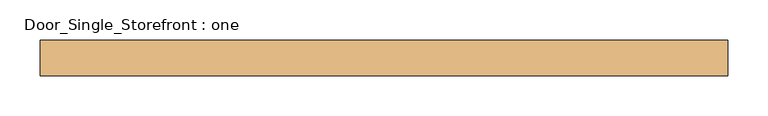
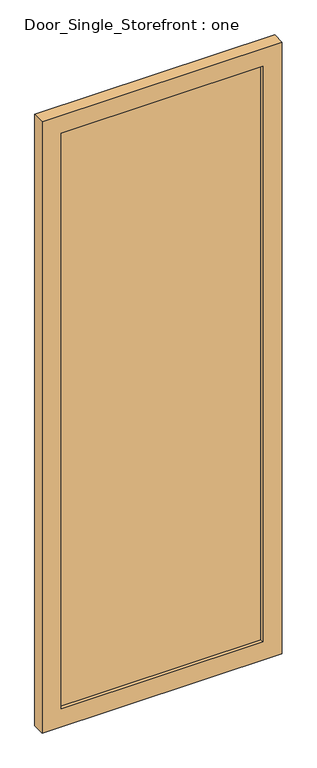
"""IFC4 building model written with IfcOpenShell, lengths in millimetres: door geometry, Door_Single_Storefront : one."""

import ifcopenshell
import ifcopenshell.guid

model = None  # the IFC model being written
_history = None  # IfcOwnerHistory: only IFC2X3 demands one
_inside = {}  # id of a spatial element -> (the spatial element, [elements in it])
_under = {}  # id of a project, library or spatial element -> (it, [spatial elements below it])
_declared = {}  # id of a project -> (the project, [libraries it declares])
_typed = {}  # id of a type object -> (the type object, [elements of that type])
_made_of = {}  # id of a material, layer set ... -> (it, [elements and type objects made of it])


def new_model(schema):
    """Start an empty IFC model of exactly this schema.

    Asked for "IFC4X3", IfcOpenShell would pick the latest addendum, in which some entities
    have other attributes; the version numbers below select the first issue.
    IFC2X3 requires an IfcOwnerHistory on every rooted entity: one is made here for all.
    """
    global model, _history
    if schema == "IFC4X3":
        model = ifcopenshell.file(schema_version=(4, 3, 0, 0))
    else:
        model = ifcopenshell.file(schema=schema)
    _inside.clear()
    _under.clear()
    _declared.clear()
    _typed.clear()
    _made_of.clear()
    _history = None
    if model.schema == "IFC2X3":
        org = make("IfcOrganization", Name="unknown")
        user = make(
            "IfcPersonAndOrganization",
            ThePerson=make("IfcPerson", FamilyName="unknown"),
            TheOrganization=org,
        )
        app = make(
            "IfcApplication",
            ApplicationDeveloper=org,
            Version="unknown",
            ApplicationFullName="unknown",
            ApplicationIdentifier="unknown",
        )
        _history = make(
            "IfcOwnerHistory",
            OwningUser=user,
            OwningApplication=app,
            ChangeAction="ADDED",
            CreationDate=0,
        )
    return model


def make(cls, **values):
    """One entity of the class cls with the attributes given. An attribute that is None is left unset."""
    return model.create_entity(
        cls, **{name: value for name, value in values.items() if value is not None}
    )


def rooted(cls, **values):
    """An entity with a GlobalId (a new one), such as an element, a storey or a relation."""
    return make(cls, GlobalId=ifcopenshell.guid.new(), OwnerHistory=_history, **values)


def si_unit(unit_type, name, prefix=None):
    """IfcSIUnit, for example si_unit("LENGTHUNIT", "METRE", prefix="MILLI")."""
    return make("IfcSIUnit", UnitType=unit_type, Prefix=prefix, Name=name)


def assignment(units):
    """IfcUnitAssignment: the units of a project."""
    return None if units is None else make("IfcUnitAssignment", Units=units)


def point(xyz):
    """IfcCartesianPoint."""
    return None if xyz is None else make("IfcCartesianPoint", Coordinates=xyz)


def direction(xyz):
    """IfcDirection."""
    return None if xyz is None else make("IfcDirection", DirectionRatios=xyz)


def frame(location, z_axis=None, x_axis=None):
    """IfcAxis2Placement3D, a coordinate frame: its origin and axes. An axis left out is left unset."""
    return make(
        "IfcAxis2Placement3D",
        Location=point(location),
        Axis=direction(z_axis),
        RefDirection=direction(x_axis),
    )


def origin():
    """The frame at (0, 0, 0) with its axes left unset."""
    return frame((0.0, 0.0, 0.0))


def place(relative_to, where):
    """IfcLocalPlacement: puts the frame where relative to a parent placement (None: the world)."""
    return make(
        "IfcLocalPlacement", PlacementRelTo=relative_to, RelativePlacement=where
    )


def context(
    kind, dimensions, precision=None, world=None, true_north=None, identifier=None
):
    """IfcGeometricRepresentationContext, for example the 3D "Model" context."""
    return make(
        "IfcGeometricRepresentationContext",
        ContextIdentifier=identifier,
        ContextType=kind,
        CoordinateSpaceDimension=dimensions,
        Precision=precision,
        WorldCoordinateSystem=world,
        TrueNorth=true_north,
    )


def project(units=None, contexts=None):
    """IfcProject with its units and contexts."""
    return rooted(
        "IfcProject",
        Name="project",
        RepresentationContexts=contexts,
        UnitsInContext=assignment(units),
    )


def spatial(cls, under=None, at=None, **own):
    """A site, building, storey or space (cls), placed at a placement, below another one or the project."""
    s = rooted(cls, ObjectPlacement=at, **own)
    if under is not None:
        _under.setdefault(under.id(), (under, []))[1].append(s)
    return s


def polyline(points):
    """IfcPolyline through the points."""
    return make("IfcPolyline", Points=[point(p) for p in points])


def outline(outer, holes=None, kind="AREA"):
    """IfcArbitraryClosedProfileDef: a profile drawn as a closed curve; with holes, ...WithVoids."""
    if holes is None:
        return make("IfcArbitraryClosedProfileDef", ProfileType=kind, OuterCurve=outer)
    return make(
        "IfcArbitraryProfileDefWithVoids",
        ProfileType=kind,
        OuterCurve=outer,
        InnerCurves=holes,
    )


def extrude(swept, where, along, depth):
    """IfcExtrudedAreaSolid: the profile swept, set in the frame where, extruded along a direction by depth."""
    return make(
        "IfcExtrudedAreaSolid",
        SweptArea=swept,
        Position=where,
        ExtrudedDirection=direction(along),
        Depth=depth,
    )


def shape(context_of_items, identifier, shape_type, items):
    """IfcShapeRepresentation: the items that make up one representation, for example the "Body"."""
    return make(
        "IfcShapeRepresentation",
        ContextOfItems=context_of_items,
        RepresentationIdentifier=identifier,
        RepresentationType=shape_type,
        Items=items,
    )


def source(mapping_origin, context_of_items, identifier, shape_type, items):
    """IfcRepresentationMap: a shape defined once, which mapped items show again and again."""
    return make(
        "IfcRepresentationMap",
        MappingOrigin=mapping_origin,
        MappedRepresentation=shape(context_of_items, identifier, shape_type, items),
    )


def transform(
    local_origin,
    x_axis=None,
    y_axis=None,
    z_axis=None,
    scale=None,
    scale2=None,
    scale3=None,
    uniform=True,
):
    """IfcCartesianTransformationOperator3D, or its non-uniform kind. x_axis, y_axis, z_axis: its Axis1, 2, 3."""
    if uniform:
        return make(
            "IfcCartesianTransformationOperator3D",
            Axis1=direction(x_axis),
            Axis2=direction(y_axis),
            LocalOrigin=point(local_origin),
            Scale=scale,
            Axis3=direction(z_axis),
        )
    return make(
        "IfcCartesianTransformationOperator3DnonUniform",
        Axis1=direction(x_axis),
        Axis2=direction(y_axis),
        LocalOrigin=point(local_origin),
        Scale=scale,
        Axis3=direction(z_axis),
        Scale2=scale2,
        Scale3=scale3,
    )


def mapped(mapping_source, mapping_target):
    """IfcMappedItem: shows the shape of a source again, moved by a transform."""
    return make(
        "IfcMappedItem", MappingSource=mapping_source, MappingTarget=mapping_target
    )


def made_of(thing, what):
    """Note that an element or type object is made of a material, layer set ...; save() writes the relation."""
    if what is not None:
        _made_of.setdefault(what.id(), (what, []))[1].append(thing)
    return thing


def element(
    cls,
    number,
    at=None,
    inside=None,
    cuts=None,
    type_object=None,
    material=None,
    context=None,
    identifier="Body",
    shape_type=None,
    held_by="IfcProductDefinitionShape",
    body=None,
    shapes=None,
    **own,
):
    """One element of the class cls, such as IfcWall. Its Tag is "e" and its number.

    at: its placement. inside: the storey or other place that contains it. cuts: it is an
    opening in that element (IfcRelVoidsElement). A single representation is given by context,
    identifier, shape_type and body (its items); several are given by shapes. held_by: the class
    of the entity that holds the representations. save() writes the other relations.
    """
    e = rooted(cls, Tag="e%d" % number, ObjectPlacement=at, **own)
    if body is not None:
        shapes = [shape(context, identifier, shape_type, body)]
    if shapes is not None:
        e.Representation = make(held_by, Representations=shapes)
    if inside is not None:
        _inside.setdefault(inside.id(), (inside, []))[1].append(e)
    if cuts is not None:
        rooted(
            "IfcRelVoidsElement", RelatingBuildingElement=cuts, RelatedOpeningElement=e
        )
    if type_object is not None:
        _typed.setdefault(type_object.id(), (type_object, []))[1].append(e)
    return made_of(e, material)


def aggregate(whole, parts):
    """IfcRelAggregates: a whole, such as a stair, and the parts it consists of."""
    return rooted("IfcRelAggregates", RelatingObject=whole, RelatedObjects=parts)


def save(model, path):
    """Write the relations noted so far, then the file.

    IfcRelAggregates (storeys below a building ...), IfcRelContainedInSpatialStructure (elements
    in a storey), IfcRelDefinesByType, IfcRelAssociatesMaterial and IfcRelDeclares: one each for
    every whole, place, type object, material and project.
    """
    for whole, parts in _under.values():
        aggregate(whole, parts)
    for where, things in _inside.values():
        rooted(
            "IfcRelContainedInSpatialStructure",
            RelatedElements=things,
            RelatingStructure=where,
        )
    for kind, things in _typed.values():
        rooted("IfcRelDefinesByType", RelatedObjects=things, RelatingType=kind)
    for what, things in _made_of.values():
        rooted("IfcRelAssociatesMaterial", RelatedObjects=things, RelatingMaterial=what)
    for by, libraries in _declared.values():
        rooted("IfcRelDeclares", RelatingContext=by, RelatedDefinitions=libraries)
    model.write(path)


def door_single_storefront_one_3727ae82(model_context):
    return source(origin(), model_context, "Body", "SweptSolid", [
        extrude(outline(polyline([(361.2994325, -6.35), (-361.2994325, -6.35), (-361.2994325, 12.7), (361.2994325, 12.7), (361.2994325, -6.35)])), frame((0.0, 0.0, 68.2625), z_axis=(0.0, 0.0, 1.0), x_axis=(1.0, 0.0, 0.0)), (0.0, 0.0, 1.0), 2176.3830968),
        extrude(outline(polyline([(2312.9080968, -429.5619325), (0.0, -429.5619325), (0.0, 429.5619325), (2312.9080968, 429.5619325), (2312.9080968, -429.5619325)]), holes=[polyline([(68.2625, 361.2994325), (68.2625, -361.2994325), (2244.6455968, -361.2994325), (2244.6455968, 361.2994325), (68.2625, 361.2994325)])]), frame((0.0, -19.05, 0.0), z_axis=(0.0, 1.0, 0.0), x_axis=(0.0, 0.0, 1.0)), (0.0, 0.0, 1.0), 44.45),
    ])


if __name__ == "__main__":
    model = new_model("IFC4")
    model_context = context("Model", 3, world=origin())
    ifc_project = project(units=[si_unit("LENGTHUNIT", "METRE", prefix="MILLI")], contexts=[model_context])
    site = spatial("IfcSite", under=ifc_project)
    building = spatial("IfcBuilding", under=site)
    placement = place(None, origin())
    door_single_storefront_one_shape = door_single_storefront_one_3727ae82(model_context)
    element("IfcDoor", 1, ObjectType="Door_Single_Storefront : one", at=placement, inside=building, context=model_context, shape_type="MappedRepresentation", body=[
        mapped(door_single_storefront_one_shape, transform((0.0, 0.0, 0.0), x_axis=(1.0, 0.0, 0.0), y_axis=(0.0, 1.0, 0.0), z_axis=(0.0, 0.0, 1.0))),
    ])
    save(model, "model.ifc")

# Revit data of these elements
# Type "Door_Single_Storefront : one"
#   Type Mark = "29"
#   OD_DS_Door_Material = "ALUM./GLAZING"
#   OD_DS_Door_Type = "STOREFRONT (NARROW STILE)"
#   OD_DS_Lockset = "ENTRY LOCK (INSIDE ADA LEVER ALWAYS ACTIVE)"
#   Analytic Construction = "<None>"
#   angle open [instance default] = 132.952°
#   Stile_Width = 0' - 2 11/16"
#   Door_Thickness = 0' - 1 3/4"
#   Door_Offset = 0' - 1"
#   Glass_Material = TEMPERED INSULATED GLAZING (CARDINAL GLASS LoĒ²-240\nOR EQUIVALENT)
#   Frame_Material = KAWNEER 260 INSULCLADTM THERMAL ENTRANCE - CLEAR ANODIZED ALUM.
#   Function = (empty or 0)
# Element 1 (IfcDoor, "Door_Single_Storefront : one")
#   angle open = 170.00°
#   Materials on its faces: "KAWNEER 260 INSULCLADTM THERMAL ENTRANCE - CLEAR ANODIZED ALUM.", "TEMPERED INSULATED GLAZING (CARDINAL GLASS LoĒ²-240\nOR EQUIVALENT)"
# Materials
#   "TEMPERED INSULATED GLAZING (CARDINAL GLASS LoĒ²-240\nOR EQUIVALENT)": class "Glass", colour RGB 196 205 210, transparency 0.85, Description = "Soda Lime Glass", Cost = 0
#   "KAWNEER 260 INSULCLADTM THERMAL ENTRANCE - CLEAR ANODIZED ALUM.": class "Metal", colour RGB 244 244 244, transparency 0, Description = "Aluminum 6061", Cost = 0
